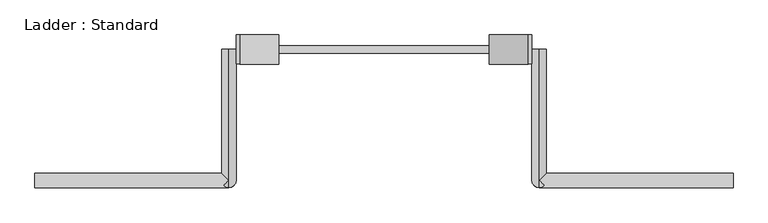
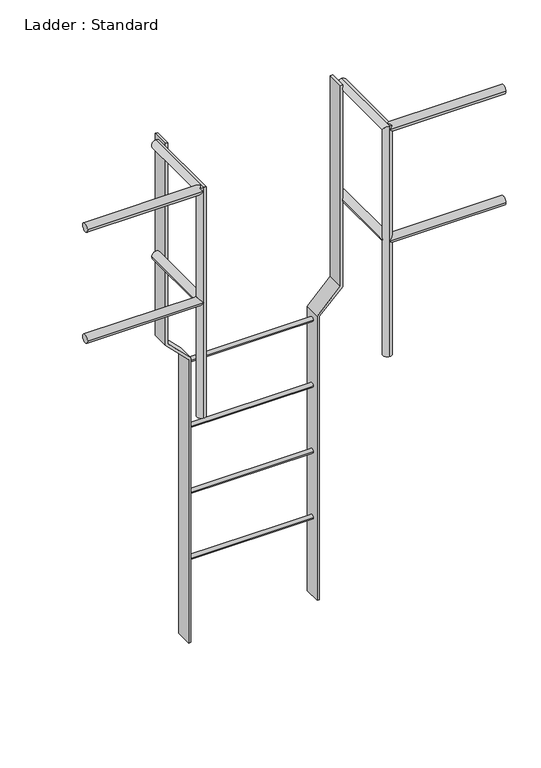
"""IFC4 building model written with IfcOpenShell, lengths in millimetres: proxy geometry, Ladder : Standard."""

import ifcopenshell
import ifcopenshell.guid

model = None  # the IFC model being written
_history = None  # IfcOwnerHistory: only IFC2X3 demands one
_inside = {}  # id of a spatial element -> (the spatial element, [elements in it])
_under = {}  # id of a project, library or spatial element -> (it, [spatial elements below it])
_declared = {}  # id of a project -> (the project, [libraries it declares])
_typed = {}  # id of a type object -> (the type object, [elements of that type])
_made_of = {}  # id of a material, layer set ... -> (it, [elements and type objects made of it])


def new_model(schema):
    """Start an empty IFC model of exactly this schema.

    Asked for "IFC4X3", IfcOpenShell would pick the latest addendum, in which some entities
    have other attributes; the version numbers below select the first issue.
    IFC2X3 requires an IfcOwnerHistory on every rooted entity: one is made here for all.
    """
    global model, _history
    if schema == "IFC4X3":
        model = ifcopenshell.file(schema_version=(4, 3, 0, 0))
    else:
        model = ifcopenshell.file(schema=schema)
    _inside.clear()
    _under.clear()
    _declared.clear()
    _typed.clear()
    _made_of.clear()
    _history = None
    if model.schema == "IFC2X3":
        org = make("IfcOrganization", Name="unknown")
        user = make(
            "IfcPersonAndOrganization",
            ThePerson=make("IfcPerson", FamilyName="unknown"),
            TheOrganization=org,
        )
        app = make(
            "IfcApplication",
            ApplicationDeveloper=org,
            Version="unknown",
            ApplicationFullName="unknown",
            ApplicationIdentifier="unknown",
        )
        _history = make(
            "IfcOwnerHistory",
            OwningUser=user,
            OwningApplication=app,
            ChangeAction="ADDED",
            CreationDate=0,
        )
    return model


def make(cls, **values):
    """One entity of the class cls with the attributes given. An attribute that is None is left unset."""
    return model.create_entity(
        cls, **{name: value for name, value in values.items() if value is not None}
    )


def rooted(cls, **values):
    """An entity with a GlobalId (a new one), such as an element, a storey or a relation."""
    return make(cls, GlobalId=ifcopenshell.guid.new(), OwnerHistory=_history, **values)


def si_unit(unit_type, name, prefix=None):
    """IfcSIUnit, for example si_unit("LENGTHUNIT", "METRE", prefix="MILLI")."""
    return make("IfcSIUnit", UnitType=unit_type, Prefix=prefix, Name=name)


def assignment(units):
    """IfcUnitAssignment: the units of a project."""
    return None if units is None else make("IfcUnitAssignment", Units=units)


def point(xyz):
    """IfcCartesianPoint."""
    return None if xyz is None else make("IfcCartesianPoint", Coordinates=xyz)


def direction(xyz):
    """IfcDirection."""
    return None if xyz is None else make("IfcDirection", DirectionRatios=xyz)


def frame(location, z_axis=None, x_axis=None):
    """IfcAxis2Placement3D, a coordinate frame: its origin and axes. An axis left out is left unset."""
    return make(
        "IfcAxis2Placement3D",
        Location=point(location),
        Axis=direction(z_axis),
        RefDirection=direction(x_axis),
    )


def frame_2d(location, x_axis=None):
    """IfcAxis2Placement2D, a coordinate frame in the plane: its origin and x axis."""
    return make(
        "IfcAxis2Placement2D", Location=point(location), RefDirection=direction(x_axis)
    )


def origin():
    """The frame at (0, 0, 0) with its axes left unset."""
    return frame((0.0, 0.0, 0.0))


def place(relative_to, where):
    """IfcLocalPlacement: puts the frame where relative to a parent placement (None: the world)."""
    return make(
        "IfcLocalPlacement", PlacementRelTo=relative_to, RelativePlacement=where
    )


def context(
    kind, dimensions, precision=None, world=None, true_north=None, identifier=None
):
    """IfcGeometricRepresentationContext, for example the 3D "Model" context."""
    return make(
        "IfcGeometricRepresentationContext",
        ContextIdentifier=identifier,
        ContextType=kind,
        CoordinateSpaceDimension=dimensions,
        Precision=precision,
        WorldCoordinateSystem=world,
        TrueNorth=true_north,
    )


def project(units=None, contexts=None):
    """IfcProject with its units and contexts."""
    return rooted(
        "IfcProject",
        Name="project",
        RepresentationContexts=contexts,
        UnitsInContext=assignment(units),
    )


def spatial(cls, under=None, at=None, **own):
    """A site, building, storey or space (cls), placed at a placement, below another one or the project."""
    s = rooted(cls, ObjectPlacement=at, **own)
    if under is not None:
        _under.setdefault(under.id(), (under, []))[1].append(s)
    return s


def polyline(points):
    """IfcPolyline through the points."""
    return make("IfcPolyline", Points=[point(p) for p in points])


def circle_curve(where, radius):
    """IfcCircle in the frame where."""
    return make("IfcCircle", Position=where, Radius=radius)


def ellipse_curve(where, semi_axis1, semi_axis2):
    """IfcEllipse in the frame where."""
    return make(
        "IfcEllipse", Position=where, SemiAxis1=semi_axis1, SemiAxis2=semi_axis2
    )


def trimmed(basis, trim1, trim2, sense, master):
    """IfcTrimmedCurve: the piece of a basis curve between two trims."""
    return make(
        "IfcTrimmedCurve",
        BasisCurve=basis,
        Trim1=trim1,
        Trim2=trim2,
        SenseAgreement=sense,
        MasterRepresentation=master,
    )


def segment(curve, same_sense, transition):
    """IfcCompositeCurveSegment."""
    return make(
        "IfcCompositeCurveSegment",
        Transition=transition,
        SameSense=same_sense,
        ParentCurve=curve,
    )


def composite_curve(segments, self_intersect=None):
    """IfcCompositeCurve: segments joined end to end."""
    return make("IfcCompositeCurve", Segments=segments, SelfIntersect=self_intersect)


def outline(outer, holes=None, kind="AREA"):
    """IfcArbitraryClosedProfileDef: a profile drawn as a closed curve; with holes, ...WithVoids."""
    if holes is None:
        return make("IfcArbitraryClosedProfileDef", ProfileType=kind, OuterCurve=outer)
    return make(
        "IfcArbitraryProfileDefWithVoids",
        ProfileType=kind,
        OuterCurve=outer,
        InnerCurves=holes,
    )


def extrude(swept, where, along, depth):
    """IfcExtrudedAreaSolid: the profile swept, set in the frame where, extruded along a direction by depth."""
    return make(
        "IfcExtrudedAreaSolid",
        SweptArea=swept,
        Position=where,
        ExtrudedDirection=direction(along),
        Depth=depth,
    )


def shape(context_of_items, identifier, shape_type, items):
    """IfcShapeRepresentation: the items that make up one representation, for example the "Body"."""
    return make(
        "IfcShapeRepresentation",
        ContextOfItems=context_of_items,
        RepresentationIdentifier=identifier,
        RepresentationType=shape_type,
        Items=items,
    )


def source(mapping_origin, context_of_items, identifier, shape_type, items):
    """IfcRepresentationMap: a shape defined once, which mapped items show again and again."""
    return make(
        "IfcRepresentationMap",
        MappingOrigin=mapping_origin,
        MappedRepresentation=shape(context_of_items, identifier, shape_type, items),
    )


def transform(
    local_origin,
    x_axis=None,
    y_axis=None,
    z_axis=None,
    scale=None,
    scale2=None,
    scale3=None,
    uniform=True,
):
    """IfcCartesianTransformationOperator3D, or its non-uniform kind. x_axis, y_axis, z_axis: its Axis1, 2, 3."""
    if uniform:
        return make(
            "IfcCartesianTransformationOperator3D",
            Axis1=direction(x_axis),
            Axis2=direction(y_axis),
            LocalOrigin=point(local_origin),
            Scale=scale,
            Axis3=direction(z_axis),
        )
    return make(
        "IfcCartesianTransformationOperator3DnonUniform",
        Axis1=direction(x_axis),
        Axis2=direction(y_axis),
        LocalOrigin=point(local_origin),
        Scale=scale,
        Axis3=direction(z_axis),
        Scale2=scale2,
        Scale3=scale3,
    )


def mapped(mapping_source, mapping_target):
    """IfcMappedItem: shows the shape of a source again, moved by a transform."""
    return make(
        "IfcMappedItem", MappingSource=mapping_source, MappingTarget=mapping_target
    )


def made_of(thing, what):
    """Note that an element or type object is made of a material, layer set ...; save() writes the relation."""
    if what is not None:
        _made_of.setdefault(what.id(), (what, []))[1].append(thing)
    return thing


def element(
    cls,
    number,
    at=None,
    inside=None,
    cuts=None,
    type_object=None,
    material=None,
    context=None,
    identifier="Body",
    shape_type=None,
    held_by="IfcProductDefinitionShape",
    body=None,
    shapes=None,
    **own,
):
    """One element of the class cls, such as IfcWall. Its Tag is "e" and its number.

    at: its placement. inside: the storey or other place that contains it. cuts: it is an
    opening in that element (IfcRelVoidsElement). A single representation is given by context,
    identifier, shape_type and body (its items); several are given by shapes. held_by: the class
    of the entity that holds the representations. save() writes the other relations.
    """
    e = rooted(cls, Tag="e%d" % number, ObjectPlacement=at, **own)
    if body is not None:
        shapes = [shape(context, identifier, shape_type, body)]
    if shapes is not None:
        e.Representation = make(held_by, Representations=shapes)
    if inside is not None:
        _inside.setdefault(inside.id(), (inside, []))[1].append(e)
    if cuts is not None:
        rooted(
            "IfcRelVoidsElement", RelatingBuildingElement=cuts, RelatedOpeningElement=e
        )
    if type_object is not None:
        _typed.setdefault(type_object.id(), (type_object, []))[1].append(e)
    return made_of(e, material)


def aggregate(whole, parts):
    """IfcRelAggregates: a whole, such as a stair, and the parts it consists of."""
    return rooted("IfcRelAggregates", RelatingObject=whole, RelatedObjects=parts)


def save(model, path):
    """Write the relations noted so far, then the file.

    IfcRelAggregates (storeys below a building ...), IfcRelContainedInSpatialStructure (elements
    in a storey), IfcRelDefinesByType, IfcRelAssociatesMaterial and IfcRelDeclares: one each for
    every whole, place, type object, material and project.
    """
    for whole, parts in _under.values():
        aggregate(whole, parts)
    for where, things in _inside.values():
        rooted(
            "IfcRelContainedInSpatialStructure",
            RelatedElements=things,
            RelatingStructure=where,
        )
    for kind, things in _typed.values():
        rooted("IfcRelDefinesByType", RelatedObjects=things, RelatingType=kind)
    for what, things in _made_of.values():
        rooted("IfcRelAssociatesMaterial", RelatedObjects=things, RelatingMaterial=what)
    for by, libraries in _declared.values():
        rooted("IfcRelDeclares", RelatingContext=by, RelatedDefinitions=libraries)
    model.write(path)


def plane_surface(at):
    """IfcPlane: the flat surface through the origin of the frame at, square to its z axis."""
    return make("IfcPlane", Position=at)


def cylinder_surface(at, radius):
    """IfcCylindricalSurface: all points at the distance radius from the z axis of the frame at."""
    return make("IfcCylindricalSurface", Position=at, Radius=radius)


def advanced_brep(points, edges, surfaces, faces):
    """IfcAdvancedBrep: a solid bounded by faces that lie on surfaces and meet in shared edges.

    An edge is (start, end): straight between two places in points (the first is 0);
    or (start, end, curve); or (start, end, curve, False) where it runs against its curve.
    A face is (place in surfaces, loops), or (place, loops, False) where it looks against
    its surface's normal. A loop lists edges by number (the first is 1), with a minus sign
    where the edge is run from its end to its start. The first loop is the outer one.
    """
    corners = [point(p) for p in points]
    vertices = [make("IfcVertexPoint", VertexGeometry=c) for c in corners]
    made = []
    for start, end, *more in edges:
        made.append(
            make(
                "IfcEdgeCurve",
                EdgeStart=vertices[start],
                EdgeEnd=vertices[end],
                EdgeGeometry=more[0] if more else make("IfcPolyline", Points=[corners[start], corners[end]]),
                SameSense=more[1] if len(more) > 1 else True,
            )
        )
    hull = []
    for where, loops, *sense in faces:
        bounds = []
        for j, loop in enumerate(loops):
            ring = [make("IfcOrientedEdge", EdgeElement=made[abs(k) - 1], Orientation=k > 0) for k in loop]
            bounds.append(
                make(
                    "IfcFaceOuterBound" if j == 0 else "IfcFaceBound",
                    Bound=make("IfcEdgeLoop", EdgeList=ring),
                    Orientation=True,
                )
            )
        hull.append(make("IfcAdvancedFace", Bounds=bounds, FaceSurface=surfaces[where], SameSense=sense[0] if sense else True))
    return make("IfcAdvancedBrep", Outer=make("IfcClosedShell", CfsFaces=hull))


def ladder_standard_509f3155(model_context):
    return source(origin(), model_context, "Body", "SolidModel", [
        extrude(outline(composite_curve([segment(trimmed(circle_curve(frame_2d((342.9, -914.4)), 9.525), [point((333.375, -914.4))], [point((352.425, -914.4))], False, "CARTESIAN"), True, "CONTINUOUS"), segment(trimmed(circle_curve(frame_2d((342.9, -914.4)), 9.525), [point((352.425, -914.4))], [point((333.375, -914.4))], False, "CARTESIAN"), True, "CONTINUOUS")], self_intersect=False)), frame((-276.3329351, 0.0, 0.0), z_axis=(1.0, 0.0, 0.0), x_axis=(0.0, 1.0, 0.0)), (0.0, 0.0, 1.0), 552.6658703),
        extrude(outline(composite_curve([segment(trimmed(circle_curve(frame_2d((342.9, -609.6)), 9.525), [point((333.375, -609.6))], [point((352.425, -609.6))], False, "CARTESIAN"), True, "CONTINUOUS"), segment(trimmed(circle_curve(frame_2d((342.9, -609.6)), 9.525), [point((352.425, -609.6))], [point((333.375, -609.6))], False, "CARTESIAN"), True, "CONTINUOUS")], self_intersect=False)), frame((-276.3329351, 0.0, 0.0), z_axis=(1.0, 0.0, 0.0), x_axis=(0.0, 1.0, 0.0)), (0.0, 0.0, 1.0), 552.6658703),
        extrude(outline(composite_curve([segment(trimmed(circle_curve(frame_2d((342.9, -304.8)), 9.525), [point((333.375, -304.8))], [point((352.425, -304.8))], False, "CARTESIAN"), True, "CONTINUOUS"), segment(trimmed(circle_curve(frame_2d((342.9, -304.8)), 9.525), [point((352.425, -304.8))], [point((333.375, -304.8))], False, "CARTESIAN"), True, "CONTINUOUS")], self_intersect=False)), frame((-276.3329351, 0.0, 0.0), z_axis=(1.0, 0.0, 0.0), x_axis=(0.0, 1.0, 0.0)), (0.0, 0.0, 1.0), 552.6658703),
        extrude(outline(composite_curve([segment(trimmed(circle_curve(frame_2d((342.9, 0.0)), 9.525), [point((333.375, 0.0))], [point((352.425, 0.0))], False, "CARTESIAN"), True, "CONTINUOUS"), segment(trimmed(circle_curve(frame_2d((342.9, 0.0)), 9.525), [point((352.425, 0.0))], [point((333.375, 0.0))], False, "CARTESIAN"), True, "CONTINUOUS")], self_intersect=False)), frame((-276.3329351, 0.0, 0.0), z_axis=(1.0, 0.0, 0.0), x_axis=(0.0, 1.0, 0.0)), (0.0, 0.0, 1.0), 552.6658703),
        advanced_brep(
        [(387.4579351, 342.9, 533.4), (425.5579351, 342.9, 533.4), (425.5579351, 19.05, 533.4), (419.9783193, 13.4703842, 519.9296158), (406.5079351, 19.05, 514.35), (387.4579351, 0.0, 533.4), (406.5079351, 19.05, 552.45), (419.9783193, 13.4703842, 546.8703842), (914.5079351, -19.05, 533.4), (914.5079351, 19.05, 533.4), (406.5079351, -19.05, 533.4), (406.5079351, 19.05, 0.0), (406.5079351, -19.05, 0.0), (406.5079351, 19.05, 1028.7), (419.9783193, 13.4703842, 1034.2796158), (406.5079351, -19.05, 1047.75), (419.9783193, -13.4703842, 1061.2203842), (406.5079351, -19.05, 1066.8), (406.5079351, 342.9, 1028.7), (406.5079351, 342.9, 1066.8), (406.5079351, 0.0, 1066.8), (425.5579351, 19.05, 1047.75), (914.5079351, -19.05, 1047.75), (914.5079351, 19.05, 1047.75)],
        [
            (0, 1, circle_curve(frame((406.5079351, 342.9, 533.4), z_axis=(0.0, 1.0, 0.0), x_axis=(1.0, 0.0, 0.0)), 19.05)),
            (1, 0, circle_curve(frame((406.5079351, 342.9, 533.4), z_axis=(0.0, 1.0, 0.0), x_axis=(1.0, 0.0, 0.0)), 19.05)),
            (1, 2),
            (2, 3, ellipse_curve(frame((406.5079351, 0.0, 533.4), z_axis=(-0.7071067811865459, 0.7071067811865492, 0.0), x_axis=(-0.7071067811865492, -0.7071067811865457, 0.0)), 26.9407684, 19.05)),
            (3, 4, ellipse_curve(frame((406.5079351, 0.0, 533.4), z_axis=(0.0, 0.7071067811865475, 0.7071067811865475), x_axis=(0.0, -0.7071067811865476, 0.7071067811865474)), 26.9407684, 19.05)),
            (4, 5, ellipse_curve(frame((406.5079351, 0.0, 533.4), z_axis=(0.0, 0.7071067811865475, 0.7071067811865475), x_axis=(0.0, -0.7071067811865476, 0.7071067811865474)), 26.9407684, 19.05)),
            (5, 0),
            (5, 6, ellipse_curve(frame((406.5079351, 0.0, 533.4), z_axis=(0.0, 0.7071067811865475, -0.7071067811865475), x_axis=(0.0, -0.7071067811865476, -0.7071067811865474)), 26.9407684, 19.05)),
            (6, 7, ellipse_curve(frame((406.5079351, 0.0, 533.4), z_axis=(0.0, 0.7071067811865475, -0.7071067811865475), x_axis=(0.0, -0.7071067811865476, -0.7071067811865474)), 26.9407684, 19.05)),
            (7, 2, ellipse_curve(frame((406.5079351, 0.0, 533.4), z_axis=(-0.7071067811865459, 0.7071067811865492, 0.0), x_axis=(-0.7071067811865492, -0.7071067811865457, 0.0)), 26.9407684, 19.05)),
            (8, 9, circle_curve(frame((914.5079351, 0.0, 533.4), z_axis=(1.0, 0.0, 0.0), x_axis=(0.0, 1.0, 0.0)), 19.05)),
            (9, 8, circle_curve(frame((914.5079351, 0.0, 533.4), z_axis=(1.0, 0.0, 0.0), x_axis=(0.0, 1.0, 0.0)), 19.05)),
            (8, 10),
            (10, 3, ellipse_curve(frame((406.5079351, 0.0, 533.4), z_axis=(0.7071067811865475, 0.0, 0.7071067811865476), x_axis=(0.7071067811865476, 0.0, -0.7071067811865474)), 26.9407684, 19.05)),
            (2, 9),
            (7, 10, ellipse_curve(frame((406.5079351, 0.0, 533.4), z_axis=(0.7071067811865476, 0.0, -0.7071067811865475), x_axis=(0.7071067811865474, 0.0, 0.7071067811865476)), 26.9407684, 19.05)),
            (11, 12, circle_curve(frame((406.5079351, 0.0, 0.0), z_axis=(0.0, 0.0, -1.0), x_axis=(0.0, -1.0, 0.0)), 19.05)),
            (12, 11, circle_curve(frame((406.5079351, 0.0, 0.0), z_axis=(0.0, 0.0, -1.0), x_axis=(0.0, -1.0, 0.0)), 19.05)),
            (11, 4),
            (10, 12),
            (6, 13),
            (13, 14, ellipse_curve(frame((406.5079351, 0.0, 1047.75), z_axis=(0.0, -0.7071067811865475, -0.7071067811865475), x_axis=(0.0, 0.7071067811865474, -0.7071067811865476)), 26.9407684, 19.05)),
            (14, 15, ellipse_curve(frame((406.5079351, 0.0, 1047.75), z_axis=(-0.7071067811865475, 0.0, -0.7071067811865476), x_axis=(0.7071067811865476, 0.0, -0.7071067811865474)), 26.9407684, 19.05)),
            (15, 10),
            (16, 17, ellipse_curve(frame((406.5079351, 0.0, 1047.75), z_axis=(0.0, -0.7071067811865475, -0.7071067811865475), x_axis=(0.0, 0.7071067811865474, -0.7071067811865476)), 26.9407684, 19.05)),
            (17, 15),
            (15, 16, ellipse_curve(frame((406.5079351, 0.0, 1047.75), z_axis=(-0.7071067811865476, 0.0, 0.7071067811865475), x_axis=(-0.7071067811865474, 0.0, -0.7071067811865476)), 26.9407684, 19.05)),
            (17, 13, ellipse_curve(frame((406.5079351, 0.0, 1047.75), z_axis=(0.0, -0.7071067811865475, -0.7071067811865475), x_axis=(0.0, 0.7071067811865474, -0.7071067811865476)), 26.9407684, 19.05)),
            (18, 19, circle_curve(frame((406.5079351, 342.9, 1047.75), z_axis=(0.0, 1.0, 0.0), x_axis=(0.0, 0.0, 1.0)), 19.05)),
            (19, 18, circle_curve(frame((406.5079351, 342.9, 1047.75), z_axis=(0.0, 1.0, 0.0), x_axis=(0.0, 0.0, 1.0)), 19.05)),
            (16, 20, ellipse_curve(frame((406.5079351, 0.0, 1047.75), z_axis=(-0.7071067811865508, -0.7071067811865441, 0.0), x_axis=(0.7071067811865441, -0.7071067811865509, 0.0)), 26.9407684, 19.05)),
            (20, 17),
            (19, 20),
            (20, 21, ellipse_curve(frame((406.5079351, 0.0, 1047.75), z_axis=(-0.7071067811865441, 0.7071067811865508, 0.0), x_axis=(-0.7071067811865507, -0.7071067811865442, 0.0)), 26.9407684, 19.05)),
            (21, 14, ellipse_curve(frame((406.5079351, 0.0, 1047.75), z_axis=(-0.7071067811865441, 0.7071067811865508, 0.0), x_axis=(-0.7071067811865507, -0.7071067811865442, 0.0)), 26.9407684, 19.05)),
            (13, 18),
            (22, 23, circle_curve(frame((914.5079351, 0.0, 1047.75), z_axis=(1.0, 0.0, 0.0), x_axis=(0.0, 1.0, 0.0)), 19.05)),
            (23, 22, circle_curve(frame((914.5079351, 0.0, 1047.75), z_axis=(1.0, 0.0, 0.0), x_axis=(0.0, 1.0, 0.0)), 19.05)),
            (22, 15),
            (21, 23),
        ],
        [
            plane_surface(frame((425.5579351, 342.9, 533.4), z_axis=(0.0, 1.0, 0.0), x_axis=(0.0, 0.0, -1.0))),
            cylinder_surface(frame((406.5079351, 342.9, 533.4), z_axis=(0.0, -1.0, 0.0), x_axis=(1.0, 0.0, 0.0)), 19.05),
            plane_surface(frame((914.5079351, 19.05, 533.4), z_axis=(1.0, 0.0, 0.0), x_axis=(0.0, 0.0, 1.0))),
            cylinder_surface(frame((406.5079351, 0.0, 533.4), z_axis=(1.0, 0.0, 0.0), x_axis=(0.0, 1.0, 0.0)), 19.05),
            plane_surface(frame((0.0, 0.0, 0.0), z_axis=(0.0, 0.0, -1.0), x_axis=(1.0, 0.0, 0.0))),
            cylinder_surface(frame((406.5079351, 0.0, 0.0), z_axis=(0.0, 0.0, -1.0), x_axis=(0.0, -1.0, 0.0)), 19.05),
            plane_surface(frame((0.0, 342.9, 1047.75), z_axis=(0.0, 1.0, 0.0), x_axis=(1.0, 0.0, 0.0))),
            cylinder_surface(frame((406.5079351, 0.0, 1047.75), z_axis=(0.0, -1.0, 0.0), x_axis=(0.0, 0.0, 1.0)), 19.05),
            plane_surface(frame((914.5079351, 19.05, 1047.75), z_axis=(1.0, 0.0, 0.0), x_axis=(0.0, 0.0, 1.0))),
            cylinder_surface(frame((406.5079351, 0.0, 1047.75), z_axis=(1.0, 0.0, 0.0), x_axis=(0.0, 1.0, 0.0)), 19.05),
        ],
        [
            (0, [[1, 2]]),
            (1, [[-2, 3, 4, 5, 6, 7]]),
            (1, [[-1, -7, 8, 9, 10, -3]]),
            (2, [[11, 12]]),
            (3, [[-11, 13, 14, -4, 15]]),
            (3, [[-12, -15, -10, 16, -13]]),
            (4, [[17, 18]]),
            (5, [[-17, 19, -5, -14, 20]]),
            (5, [[21, 22, 23, 24, -16, -9]]),
            (5, [[25, 26, 27]]),
            (5, [[-18, -20, -24, -26, 28, -21, -8, -6, -19]]),
            (6, [[29, 30]]),
            (7, [[-25, 31, 32]]),
            (7, [[-30, 33, 34, 35, -22, 36]]),
            (7, [[-28, -32, -33, -29, -36]]),
            (8, [[37, 38]]),
            (9, [[-37, 39, -23, -35, 40]]),
            (9, [[-38, -40, -34, -31, -27, -39]]),
        ],
    ),
        advanced_brep(
        [(-914.5079351, -19.05, 533.4), (-914.5079351, 19.05, 533.4), (-425.5579351, 19.05, 533.4), (-419.9783193, 13.4703842, 519.9296158), (-406.5079351, -19.05, 533.4), (-419.9783193, 13.4703842, 546.8703842), (-425.5579351, 342.9, 533.4), (-387.4579351, 342.9, 533.4), (-387.4579351, 0.0, 533.4), (-406.5079351, 19.05, 514.35), (-406.5079351, 19.05, 552.45), (-406.5079351, 19.05, 0.0), (-406.5079351, -19.05, 0.0), (-406.5079351, 19.05, 1028.7), (-406.5079351, -19.05, 1066.8), (-406.5079351, -19.05, 1047.75), (-419.9783193, 13.4703842, 1034.2796158), (-419.9783193, -13.4703842, 1061.2203842), (-406.5079351, 342.9, 1028.7), (-406.5079351, 342.9, 1066.8), (-406.5079351, 0.0, 1066.8), (-425.5579351, 19.05, 1047.75), (-914.5079351, -19.05, 1047.75), (-914.5079351, 19.05, 1047.75)],
        [
            (0, 1, circle_curve(frame((-914.5079351, 0.0, 533.4), z_axis=(-1.0, 0.0, 0.0), x_axis=(0.0, 1.0, 0.0)), 19.05)),
            (1, 0, circle_curve(frame((-914.5079351, 0.0, 533.4), z_axis=(-1.0, 0.0, 0.0), x_axis=(0.0, 1.0, 0.0)), 19.05)),
            (1, 2),
            (2, 3, ellipse_curve(frame((-406.5079351, 0.0, 533.4), z_axis=(-0.7071067811865491, -0.7071067811865458, 0.0), x_axis=(0.7071067811865459, -0.707106781186549, 0.0)), 26.9407684, 19.05)),
            (3, 4, ellipse_curve(frame((-406.5079351, 0.0, 533.4), z_axis=(-0.7071067811865476, 0.0, 0.7071067811865475), x_axis=(0.7071067811865474, 0.0, 0.7071067811865476)), 26.9407684, 19.05)),
            (4, 0),
            (4, 5, ellipse_curve(frame((-406.5079351, 0.0, 533.4), z_axis=(-0.7071067811865475, 0.0, -0.7071067811865476), x_axis=(0.7071067811865476, 0.0, -0.7071067811865474)), 26.9407684, 19.05)),
            (5, 2, ellipse_curve(frame((-406.5079351, 0.0, 533.4), z_axis=(-0.7071067811865491, -0.7071067811865458, 0.0), x_axis=(0.7071067811865459, -0.707106781186549, 0.0)), 26.9407684, 19.05)),
            (6, 7, circle_curve(frame((-406.5079351, 342.9, 533.4), z_axis=(0.0, 1.0, 0.0), x_axis=(1.0, 0.0, 0.0)), 19.05)),
            (7, 6, circle_curve(frame((-406.5079351, 342.9, 533.4), z_axis=(0.0, 1.0, 0.0), x_axis=(1.0, 0.0, 0.0)), 19.05)),
            (7, 8),
            (8, 9, ellipse_curve(frame((-406.5079351, 0.0, 533.4), z_axis=(0.0, 0.7071067811865475, 0.7071067811865475), x_axis=(0.0, -0.7071067811865476, 0.7071067811865474)), 26.9407684, 19.05)),
            (9, 3, ellipse_curve(frame((-406.5079351, 0.0, 533.4), z_axis=(0.0, 0.7071067811865475, 0.7071067811865475), x_axis=(0.0, -0.7071067811865476, 0.7071067811865474)), 26.9407684, 19.05)),
            (2, 6),
            (5, 10, ellipse_curve(frame((-406.5079351, 0.0, 533.4), z_axis=(0.0, 0.7071067811865475, -0.7071067811865475), x_axis=(0.0, -0.7071067811865476, -0.7071067811865474)), 26.9407684, 19.05)),
            (10, 8, ellipse_curve(frame((-406.5079351, 0.0, 533.4), z_axis=(0.0, 0.7071067811865475, -0.7071067811865475), x_axis=(0.0, -0.7071067811865476, -0.7071067811865474)), 26.9407684, 19.05)),
            (11, 12, circle_curve(frame((-406.5079351, 0.0, 0.0), z_axis=(0.0, 0.0, -1.0), x_axis=(0.0, -1.0, 0.0)), 19.05)),
            (12, 11, circle_curve(frame((-406.5079351, 0.0, 0.0), z_axis=(0.0, 0.0, -1.0), x_axis=(0.0, -1.0, 0.0)), 19.05)),
            (11, 9),
            (10, 13),
            (13, 14, ellipse_curve(frame((-406.5079351, 0.0, 1047.75), z_axis=(0.0, -0.7071067811865475, -0.7071067811865475), x_axis=(0.0, 0.7071067811865474, -0.7071067811865476)), 26.9407684, 19.05)),
            (14, 15),
            (15, 4),
            (4, 12),
            (15, 16, ellipse_curve(frame((-406.5079351, 0.0, 1047.75), z_axis=(0.7071067811865476, 0.0, -0.7071067811865475), x_axis=(-0.7071067811865474, 0.0, -0.7071067811865476)), 26.9407684, 19.05)),
            (16, 13, ellipse_curve(frame((-406.5079351, 0.0, 1047.75), z_axis=(0.0, -0.7071067811865475, -0.7071067811865475), x_axis=(0.0, 0.7071067811865474, -0.7071067811865476)), 26.9407684, 19.05)),
            (14, 17, ellipse_curve(frame((-406.5079351, 0.0, 1047.75), z_axis=(0.0, -0.7071067811865475, -0.7071067811865475), x_axis=(0.0, 0.7071067811865474, -0.7071067811865476)), 26.9407684, 19.05)),
            (17, 15, ellipse_curve(frame((-406.5079351, 0.0, 1047.75), z_axis=(0.7071067811865475, 0.0, 0.7071067811865476), x_axis=(0.7071067811865476, 0.0, -0.7071067811865474)), 26.9407684, 19.05)),
            (18, 19, circle_curve(frame((-406.5079351, 342.9, 1047.75), z_axis=(0.0, 1.0, 0.0), x_axis=(0.0, 0.0, 1.0)), 19.05)),
            (19, 18, circle_curve(frame((-406.5079351, 342.9, 1047.75), z_axis=(0.0, 1.0, 0.0), x_axis=(0.0, 0.0, 1.0)), 19.05)),
            (13, 18),
            (19, 20),
            (20, 14),
            (20, 17, ellipse_curve(frame((-406.5079351, 0.0, 1047.75), z_axis=(0.7071067811865441, -0.7071067811865508, 0.0), x_axis=(-0.7071067811865507, -0.7071067811865442, 0.0)), 26.9407684, 19.05)),
            (16, 21, ellipse_curve(frame((-406.5079351, 0.0, 1047.75), z_axis=(0.7071067811865508, 0.7071067811865441, 0.0), x_axis=(0.7071067811865441, -0.7071067811865509, 0.0)), 26.9407684, 19.05)),
            (21, 20, ellipse_curve(frame((-406.5079351, 0.0, 1047.75), z_axis=(0.7071067811865508, 0.7071067811865441, 0.0), x_axis=(0.7071067811865441, -0.7071067811865509, 0.0)), 26.9407684, 19.05)),
            (22, 23, circle_curve(frame((-914.5079351, 0.0, 1047.75), z_axis=(-1.0, 0.0, 0.0), x_axis=(0.0, 1.0, 0.0)), 19.05)),
            (23, 22, circle_curve(frame((-914.5079351, 0.0, 1047.75), z_axis=(-1.0, 0.0, 0.0), x_axis=(0.0, 1.0, 0.0)), 19.05)),
            (23, 21),
            (15, 22),
        ],
        [
            plane_surface(frame((-914.5079351, 19.05, 533.4), z_axis=(-1.0, 0.0, 0.0), x_axis=(0.0, 0.0, -1.0))),
            cylinder_surface(frame((-914.5079351, 0.0, 533.4), z_axis=(1.0, 0.0, 0.0), x_axis=(0.0, 1.0, 0.0)), 19.05),
            plane_surface(frame((-387.4579351, 342.9, 533.4), z_axis=(0.0, 1.0, 0.0), x_axis=(0.0, 0.0, -1.0))),
            cylinder_surface(frame((-406.5079351, 342.9, 533.4), z_axis=(0.0, -1.0, 0.0), x_axis=(1.0, 0.0, 0.0)), 19.05),
            plane_surface(frame((0.0, 0.0, 0.0), z_axis=(0.0, 0.0, -1.0), x_axis=(1.0, 0.0, 0.0))),
            cylinder_surface(frame((-406.5079351, 0.0, 0.0), z_axis=(0.0, 0.0, -1.0), x_axis=(0.0, -1.0, 0.0)), 19.05),
            plane_surface(frame((0.0, 342.9, 1047.75), z_axis=(0.0, 1.0, 0.0), x_axis=(1.0, 0.0, 0.0))),
            cylinder_surface(frame((-406.5079351, 0.0, 1047.75), z_axis=(0.0, -1.0, 0.0), x_axis=(0.0, 0.0, 1.0)), 19.05),
            plane_surface(frame((-914.5079351, 19.05, 1047.75), z_axis=(-1.0, 0.0, 0.0), x_axis=(0.0, 0.0, -1.0))),
            cylinder_surface(frame((-914.5079351, 0.0, 1047.75), z_axis=(1.0, 0.0, 0.0), x_axis=(0.0, 1.0, 0.0)), 19.05),
        ],
        [
            (0, [[1, 2]]),
            (1, [[-2, 3, 4, 5, 6]]),
            (1, [[-1, -6, 7, 8, -3]]),
            (2, [[9, 10]]),
            (3, [[-10, 11, 12, 13, -4, 14]]),
            (3, [[-9, -14, -8, 15, 16, -11]]),
            (4, [[17, 18]]),
            (5, [[-17, 19, -12, -16, 20, 21, 22, 23, 24]]),
            (5, [[-18, -24, -5, -13, -19]]),
            (5, [[-20, -15, -7, -23, 25, 26]]),
            (5, [[27, 28, -22]]),
            (6, [[29, 30]]),
            (7, [[-21, 31, -30, 32, 33]]),
            (7, [[-27, -33, 34]]),
            (7, [[-29, -31, -26, 35, 36, -32]]),
            (8, [[37, 38]]),
            (9, [[-38, 39, -35, -25, 40]]),
            (9, [[-37, -40, -28, -34, -36, -39]]),
        ],
    ),
        extrude(outline(polyline([(1066.8, -387.4579351), (133.35, -387.4579351), (31.75, -285.8579351), (-1279.5743936, -285.8579351), (-1279.5743936, -276.3329351), (35.6953842, -276.3329351), (137.2953842, -377.9329351), (1066.8, -377.9329351), (1066.8, -387.4579351)])), frame((0.0, 304.8, 0.0), z_axis=(0.0, 1.0, 0.0), x_axis=(0.0, 0.0, 1.0)), (0.0, 0.0, 1.0), 76.2),
        extrude(outline(polyline([(1066.8, 377.9329351), (137.2953842, 377.9329351), (35.6953842, 276.3329351), (-1279.5743936, 276.3329351), (-1279.5743936, 285.8579351), (31.75, 285.8579351), (133.35, 387.4579351), (1066.8, 387.4579351), (1066.8, 377.9329351)])), frame((0.0, 304.8, 0.0), z_axis=(0.0, 1.0, 0.0), x_axis=(0.0, 0.0, 1.0)), (0.0, 0.0, 1.0), 76.2),
    ])


if __name__ == "__main__":
    model = new_model("IFC4")
    model_context = context("Model", 3, world=origin())
    ifc_project = project(units=[si_unit("LENGTHUNIT", "METRE", prefix="MILLI")], contexts=[model_context])
    site = spatial("IfcSite", under=ifc_project)
    building = spatial("IfcBuilding", under=site)
    placement = place(None, origin())
    ladder_standard_shape = ladder_standard_509f3155(model_context)
    element("IfcBuildingElementProxy", 1, Name="Ladder : Standard", ObjectType="Ladder : Standard", at=placement, inside=building, context=model_context, shape_type="MappedRepresentation", body=[
        mapped(ladder_standard_shape, transform((0.0, 0.0, 0.0), x_axis=(1.0, 0.0, 0.0), y_axis=(0.0, 1.0, 0.0), z_axis=(0.0, 0.0, 1.0))),
    ])
    save(model, "model.ifc")

# Revit data of these elements
# Type "Ladder : Standard"
#   Rung Radius = 9.525 mm
#   Rung Length [instance default] = 406.4 mm
#   Side Rail Thickness = 76.2 mm
#   Side Rail Width = 9.525 mm
#   Half Guardrail Height = 533.4 mm
#   Height [instance default] = 4635.5 mm
#   Guardrail Length = 508 mm
#   Guardrail Height = 1066.8 mm
#   Distance [instance default] = 177.8 mm
#   Rung Space [instance default] = 304.8 mm
#   Number of Rungs [instance default] = 15
#   Default Elevation = 0
# Element 1 (IfcBuildingElementProxy, "Ladder : Standard")
#   Rung Length = 552.666 mm
#   Height = 1279.574 mm
#   Number of Rungs = 4
